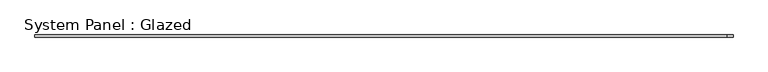
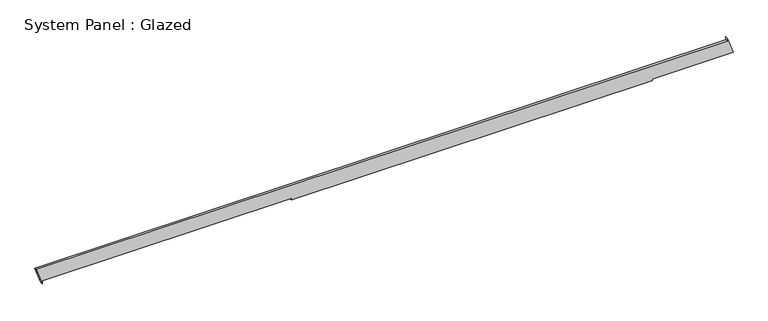
"""IFC4 building model written with IfcOpenShell, lengths in millimetres: plate geometry, System Panel : Glazed."""

import ifcopenshell
import ifcopenshell.guid

model = None  # the IFC model being written
_history = None  # IfcOwnerHistory: only IFC2X3 demands one
_inside = {}  # id of a spatial element -> (the spatial element, [elements in it])
_under = {}  # id of a project, library or spatial element -> (it, [spatial elements below it])
_declared = {}  # id of a project -> (the project, [libraries it declares])
_typed = {}  # id of a type object -> (the type object, [elements of that type])
_made_of = {}  # id of a material, layer set ... -> (it, [elements and type objects made of it])


def new_model(schema):
    """Start an empty IFC model of exactly this schema.

    Asked for "IFC4X3", IfcOpenShell would pick the latest addendum, in which some entities
    have other attributes; the version numbers below select the first issue.
    IFC2X3 requires an IfcOwnerHistory on every rooted entity: one is made here for all.
    """
    global model, _history
    if schema == "IFC4X3":
        model = ifcopenshell.file(schema_version=(4, 3, 0, 0))
    else:
        model = ifcopenshell.file(schema=schema)
    _inside.clear()
    _under.clear()
    _declared.clear()
    _typed.clear()
    _made_of.clear()
    _history = None
    if model.schema == "IFC2X3":
        org = make("IfcOrganization", Name="unknown")
        user = make(
            "IfcPersonAndOrganization",
            ThePerson=make("IfcPerson", FamilyName="unknown"),
            TheOrganization=org,
        )
        app = make(
            "IfcApplication",
            ApplicationDeveloper=org,
            Version="unknown",
            ApplicationFullName="unknown",
            ApplicationIdentifier="unknown",
        )
        _history = make(
            "IfcOwnerHistory",
            OwningUser=user,
            OwningApplication=app,
            ChangeAction="ADDED",
            CreationDate=0,
        )
    return model


def make(cls, **values):
    """One entity of the class cls with the attributes given. An attribute that is None is left unset."""
    return model.create_entity(
        cls, **{name: value for name, value in values.items() if value is not None}
    )


def rooted(cls, **values):
    """An entity with a GlobalId (a new one), such as an element, a storey or a relation."""
    return make(cls, GlobalId=ifcopenshell.guid.new(), OwnerHistory=_history, **values)


def si_unit(unit_type, name, prefix=None):
    """IfcSIUnit, for example si_unit("LENGTHUNIT", "METRE", prefix="MILLI")."""
    return make("IfcSIUnit", UnitType=unit_type, Prefix=prefix, Name=name)


def assignment(units):
    """IfcUnitAssignment: the units of a project."""
    return None if units is None else make("IfcUnitAssignment", Units=units)


def point(xyz):
    """IfcCartesianPoint."""
    return None if xyz is None else make("IfcCartesianPoint", Coordinates=xyz)


def direction(xyz):
    """IfcDirection."""
    return None if xyz is None else make("IfcDirection", DirectionRatios=xyz)


def frame(location, z_axis=None, x_axis=None):
    """IfcAxis2Placement3D, a coordinate frame: its origin and axes. An axis left out is left unset."""
    return make(
        "IfcAxis2Placement3D",
        Location=point(location),
        Axis=direction(z_axis),
        RefDirection=direction(x_axis),
    )


def origin():
    """The frame at (0, 0, 0) with its axes left unset."""
    return frame((0.0, 0.0, 0.0))


def place(relative_to, where):
    """IfcLocalPlacement: puts the frame where relative to a parent placement (None: the world)."""
    return make(
        "IfcLocalPlacement", PlacementRelTo=relative_to, RelativePlacement=where
    )


def context(
    kind, dimensions, precision=None, world=None, true_north=None, identifier=None
):
    """IfcGeometricRepresentationContext, for example the 3D "Model" context."""
    return make(
        "IfcGeometricRepresentationContext",
        ContextIdentifier=identifier,
        ContextType=kind,
        CoordinateSpaceDimension=dimensions,
        Precision=precision,
        WorldCoordinateSystem=world,
        TrueNorth=true_north,
    )


def project(units=None, contexts=None):
    """IfcProject with its units and contexts."""
    return rooted(
        "IfcProject",
        Name="project",
        RepresentationContexts=contexts,
        UnitsInContext=assignment(units),
    )


def spatial(cls, under=None, at=None, **own):
    """A site, building, storey or space (cls), placed at a placement, below another one or the project."""
    s = rooted(cls, ObjectPlacement=at, **own)
    if under is not None:
        _under.setdefault(under.id(), (under, []))[1].append(s)
    return s


def polyline(points):
    """IfcPolyline through the points."""
    return make("IfcPolyline", Points=[point(p) for p in points])


def outline(outer, holes=None, kind="AREA"):
    """IfcArbitraryClosedProfileDef: a profile drawn as a closed curve; with holes, ...WithVoids."""
    if holes is None:
        return make("IfcArbitraryClosedProfileDef", ProfileType=kind, OuterCurve=outer)
    return make(
        "IfcArbitraryProfileDefWithVoids",
        ProfileType=kind,
        OuterCurve=outer,
        InnerCurves=holes,
    )


def extrude(swept, where, along, depth):
    """IfcExtrudedAreaSolid: the profile swept, set in the frame where, extruded along a direction by depth."""
    return make(
        "IfcExtrudedAreaSolid",
        SweptArea=swept,
        Position=where,
        ExtrudedDirection=direction(along),
        Depth=depth,
    )


def shape(context_of_items, identifier, shape_type, items):
    """IfcShapeRepresentation: the items that make up one representation, for example the "Body"."""
    return make(
        "IfcShapeRepresentation",
        ContextOfItems=context_of_items,
        RepresentationIdentifier=identifier,
        RepresentationType=shape_type,
        Items=items,
    )


def source(mapping_origin, context_of_items, identifier, shape_type, items):
    """IfcRepresentationMap: a shape defined once, which mapped items show again and again."""
    return make(
        "IfcRepresentationMap",
        MappingOrigin=mapping_origin,
        MappedRepresentation=shape(context_of_items, identifier, shape_type, items),
    )


def transform(
    local_origin,
    x_axis=None,
    y_axis=None,
    z_axis=None,
    scale=None,
    scale2=None,
    scale3=None,
    uniform=True,
):
    """IfcCartesianTransformationOperator3D, or its non-uniform kind. x_axis, y_axis, z_axis: its Axis1, 2, 3."""
    if uniform:
        return make(
            "IfcCartesianTransformationOperator3D",
            Axis1=direction(x_axis),
            Axis2=direction(y_axis),
            LocalOrigin=point(local_origin),
            Scale=scale,
            Axis3=direction(z_axis),
        )
    return make(
        "IfcCartesianTransformationOperator3DnonUniform",
        Axis1=direction(x_axis),
        Axis2=direction(y_axis),
        LocalOrigin=point(local_origin),
        Scale=scale,
        Axis3=direction(z_axis),
        Scale2=scale2,
        Scale3=scale3,
    )


def mapped(mapping_source, mapping_target):
    """IfcMappedItem: shows the shape of a source again, moved by a transform."""
    return make(
        "IfcMappedItem", MappingSource=mapping_source, MappingTarget=mapping_target
    )


def made_of(thing, what):
    """Note that an element or type object is made of a material, layer set ...; save() writes the relation."""
    if what is not None:
        _made_of.setdefault(what.id(), (what, []))[1].append(thing)
    return thing


def element(
    cls,
    number,
    at=None,
    inside=None,
    cuts=None,
    type_object=None,
    material=None,
    context=None,
    identifier="Body",
    shape_type=None,
    held_by="IfcProductDefinitionShape",
    body=None,
    shapes=None,
    **own,
):
    """One element of the class cls, such as IfcWall. Its Tag is "e" and its number.

    at: its placement. inside: the storey or other place that contains it. cuts: it is an
    opening in that element (IfcRelVoidsElement). A single representation is given by context,
    identifier, shape_type and body (its items); several are given by shapes. held_by: the class
    of the entity that holds the representations. save() writes the other relations.
    """
    e = rooted(cls, Tag="e%d" % number, ObjectPlacement=at, **own)
    if body is not None:
        shapes = [shape(context, identifier, shape_type, body)]
    if shapes is not None:
        e.Representation = make(held_by, Representations=shapes)
    if inside is not None:
        _inside.setdefault(inside.id(), (inside, []))[1].append(e)
    if cuts is not None:
        rooted(
            "IfcRelVoidsElement", RelatingBuildingElement=cuts, RelatedOpeningElement=e
        )
    if type_object is not None:
        _typed.setdefault(type_object.id(), (type_object, []))[1].append(e)
    return made_of(e, material)


def aggregate(whole, parts):
    """IfcRelAggregates: a whole, such as a stair, and the parts it consists of."""
    return rooted("IfcRelAggregates", RelatingObject=whole, RelatedObjects=parts)


def save(model, path):
    """Write the relations noted so far, then the file.

    IfcRelAggregates (storeys below a building ...), IfcRelContainedInSpatialStructure (elements
    in a storey), IfcRelDefinesByType, IfcRelAssociatesMaterial and IfcRelDeclares: one each for
    every whole, place, type object, material and project.
    """
    for whole, parts in _under.values():
        aggregate(whole, parts)
    for where, things in _inside.values():
        rooted(
            "IfcRelContainedInSpatialStructure",
            RelatedElements=things,
            RelatingStructure=where,
        )
    for kind, things in _typed.values():
        rooted("IfcRelDefinesByType", RelatedObjects=things, RelatingType=kind)
    for what, things in _made_of.values():
        rooted("IfcRelAssociatesMaterial", RelatedObjects=things, RelatingMaterial=what)
    for by, libraries in _declared.values():
        rooted("IfcRelDeclares", RelatingContext=by, RelatedDefinitions=libraries)
    model.write(path)


def system_panel_glazed_82b7ec84(model_context):
    return source(origin(), model_context, "Body", "SweptSolid", [
        extrude(outline(polyline([(0.0, -3959.3382367), (35.3553391, -3959.3382367), (35.3553391, -1080.0643239), (19.2141513, -1079.589913), (19.2159629, 3093.0829852), (35.3553391, 3094.3752998), (35.3553391, 4027.9814555), (234.8084044, 3959.4408873), (199.4530653, 3959.4410749), (199.4106846, -4027.9814555), (0.0, -3959.3382367)])), frame((0.0, -49.5, 0.0), z_axis=(0.0, 1.0, 0.0), x_axis=(0.0, 0.0, 1.0)), (0.0, 0.0, 1.0), 25.0),
    ])


if __name__ == "__main__":
    model = new_model("IFC4")
    model_context = context("Model", 3, world=origin())
    ifc_project = project(units=[si_unit("LENGTHUNIT", "METRE", prefix="MILLI")], contexts=[model_context])
    site = spatial("IfcSite", under=ifc_project)
    building = spatial("IfcBuilding", under=site)
    placement = place(None, origin())
    system_panel_glazed_shape = system_panel_glazed_82b7ec84(model_context)
    element("IfcPlate", 1, ObjectType="System Panel : Glazed", at=placement, inside=building, context=model_context, shape_type="MappedRepresentation", body=[
        mapped(system_panel_glazed_shape, transform((0.0, 0.0, 0.0), x_axis=(1.0, 0.0, 0.0), y_axis=(0.0, 1.0, 0.0), z_axis=(0.0, 0.0, 1.0))),
    ])
    save(model, "model.ifc")

# Revit data of these elements
# Element 1 (IfcPlate, "System Panel : Glazed")
#   Materials on its faces: "Glass"
# Materials
#   "Glass": class "Glass", colour RGB 218 227 224, transparency 0.85, Description = "Soda Lime Glass", Cost = 0
